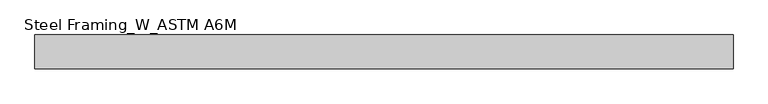
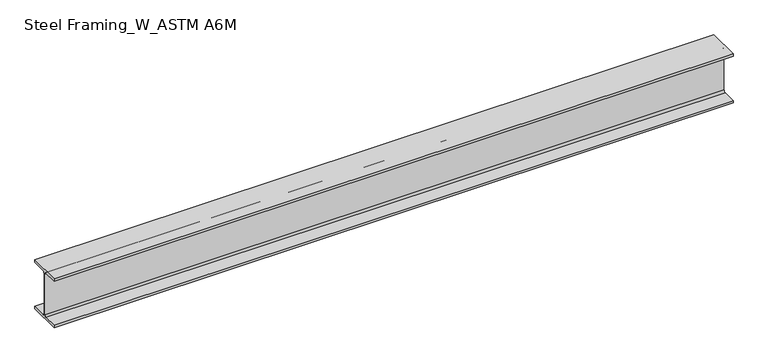
"""IFC4 building model written with IfcOpenShell, lengths in millimetres: beam geometry, Steel Framing_W_ASTM A6M : H_SB_AR_S02_W200x31.3_B6."""

from ifc_helpers import new_model, si_unit, point, frame, frame_2d, origin, place, context, project, spatial, polyline, circle_curve, trimmed, segment, composite_curve, outline, extrude, source, transform, mapped, element, save


def steel_framing_w_astm_a6m_fa6438b5(model_context):
    return source(origin(), model_context, "Body", "SweptSolid", [
        extrude(outline(composite_curve([segment(polyline([(67.0, -94.8), (67.0, -105.0), (-67.0, -105.0), (-67.0, -94.8), (-10.775, -94.8)]), True, "CONTINUOUS"), segment(trimmed(circle_curve(frame_2d((-10.775, -87.2)), 7.6), [point((-10.775, -94.8))], [point((-3.175, -87.2))], True, "CARTESIAN"), True, "CONTINUOUS"), segment(polyline([(-3.175, -87.2), (-3.175, 87.2)]), True, "CONTINUOUS"), segment(trimmed(circle_curve(frame_2d((-10.775, 87.2)), 7.6), [point((-3.175, 87.2))], [point((-10.775, 94.8))], True, "CARTESIAN"), True, "CONTINUOUS"), segment(polyline([(-10.775, 94.8), (-67.0, 94.8), (-67.0, 105.0), (67.0, 105.0), (67.0, 94.8), (10.775, 94.8)]), True, "CONTINUOUS"), segment(trimmed(circle_curve(frame_2d((10.775, 87.2)), 7.6), [point((10.775, 94.8))], [point((3.175, 87.2))], True, "CARTESIAN"), True, "CONTINUOUS"), segment(polyline([(3.175, 87.2), (3.175, -87.2)]), True, "CONTINUOUS"), segment(trimmed(circle_curve(frame_2d((10.775, -87.2)), 7.6), [point((3.175, -87.2))], [point((10.775, -94.8))], True, "CARTESIAN"), True, "CONTINUOUS"), segment(polyline([(10.775, -94.8), (67.0, -94.8)]), True, "CONTINUOUS")], self_intersect=False)), frame((-1350.0, 0.0, 0.0), z_axis=(1.0, 0.0, 0.0), x_axis=(0.0, 1.0, 0.0)), (0.0, 0.0, 1.0), 2751.8),
    ])


if __name__ == "__main__":
    model = new_model("IFC4")
    model_context = context("Model", 3, world=origin())
    ifc_project = project(units=[si_unit("LENGTHUNIT", "METRE", prefix="MILLI")], contexts=[model_context])
    site = spatial("IfcSite", under=ifc_project)
    building = spatial("IfcBuilding", under=site)
    placement = place(None, origin())
    steel_framing_w_astm_a6m_shape = steel_framing_w_astm_a6m_fa6438b5(model_context)
    element("IfcBeam", 1, ObjectType="Steel Framing_W_ASTM A6M : H_SB_AR_S02_W200x31.3_B6", at=placement, inside=building, context=model_context, shape_type="MappedRepresentation", body=[
        mapped(steel_framing_w_astm_a6m_shape, transform((0.0, 0.0, 0.0), x_axis=(1.0, 0.0, 0.0), y_axis=(0.0, 1.0, 0.0), z_axis=(0.0, 0.0, 1.0))),
    ])
    save(model, "model.ifc")

# Revit data of these elements
# Type "Steel Framing_W_ASTM A6M : H_SB_AR_S02_W200x31.3_B6"
#   Type Mark = "B6"
#   Section Name Key = "W8x21"
#   Width = 13.4 cm
#   Web Thickness = 0.635 cm
#   Web Fillet = 0.76 cm
#   Warping Constant = 40800.0 cm⁶
#   Torsional Moment of Inertia = 11.70 cm⁴
#   Section Area = 39.7 cm²
#   Plastic Modulus weak axis = 93.2 cm³
#   Plastic Modulus strong axis = 334.0 cm³
#   Perimeter = 0.93 m²/m
#   Nominal Weight = 31.30 kgf/m
#   Moment of Inertia weak axis = 407.00 cm⁴
#   Moment of Inertia strong axis = 3130.00 cm⁴
#   Height = 21.0 cm
#   Flange Thickness = 1.02 cm
#   Elastic Modulus weak axis = 60.8 cm³
#   Elastic Modulus strong axis = 298.0 cm³
#   Centroid Vertical = 10.5 cm
#   Centroid Horizontal = 6.7 cm
#   Length [instance default] = 1500 mm
#   Structural Material [instance default] = Steel, 45-345
#   Bolt Spacing = 0
#   Assembly Code = ""
# Element 1 (IfcBeam, "Steel Framing_W_ASTM A6M : H_SB_AR_S02_W200x31.3_B6")
#   Materials on its faces: "Steel, 45-345"
# Materials
#   "Steel, 45-345": class "Metal", colour RGB 189 187 185, transparency 0, Description = "Steel 345 MPa", Cost = 0
